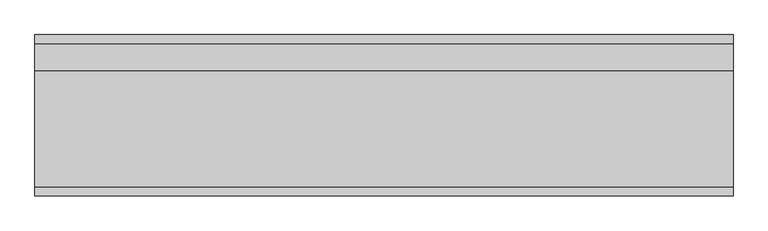
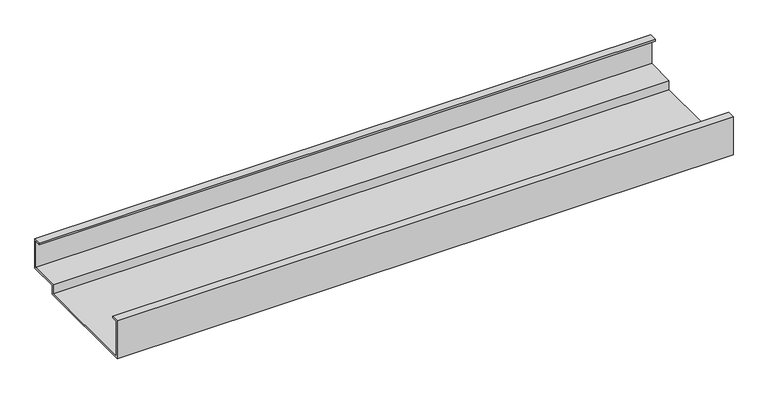
"""IFC4 building model written with IfcOpenShell, lengths in millimetres: proxy geometry, Generic Models 7:Generic Models 1:337419:Generic Models 1:337419 : Generic Models 7:Generic Models 1:337419:13 : Generic Models 7:Generic Models 1:337419:Generic Models 1:337419 : Generic Models 7:Generic Models 1:337419:301336."""

from ifc_helpers import new_model, si_unit, frame, origin, place, context, project, spatial, polyline, outline, extrude, source, transform, mapped, element, save


def generic_models_601f3d41(model_context):
    return source(origin(), model_context, "Body", "SweptSolid", [
        extrude(outline(polyline([(-536557.2913358, 2489.2), (-536557.2913358, 2438.4), (-536606.5038358, 2438.4), (-536606.5038358, 2422.525), (-536792.2413358, 2422.525), (-536792.2413358, 2489.2), (-536779.5413358, 2489.2), (-536779.5413358, 2486.421875), (-536789.4632108, 2486.421875), (-536789.4632108, 2425.303125), (-536609.2819608, 2425.303125), (-536609.2819608, 2441.178125), (-536560.0694608, 2441.178125), (-536560.0694608, 2486.421875), (-536569.9913358, 2486.421875), (-536569.9913358, 2489.2), (-536557.2913358, 2489.2)])), frame((592715.7367242, 0.0, 0.0), z_axis=(1.0, 0.0, 0.0), x_axis=(0.0, 1.0, 0.0)), (0.0, 0.0, 1.0), 1016.0),
    ])


if __name__ == "__main__":
    model = new_model("IFC4")
    model_context = context("Model", 3, world=origin())
    ifc_project = project(units=[si_unit("LENGTHUNIT", "METRE", prefix="MILLI")], contexts=[model_context])
    site = spatial("IfcSite", under=ifc_project)
    building = spatial("IfcBuilding", under=site)
    placement = place(None, origin())
    generic_models_shape = generic_models_601f3d41(model_context)
    element("IfcBuildingElementProxy", 1, Name="Generic Models 7:Generic Models 1:337419:Generic Models 1:337419 : Generic Models 7:Generic Models 1:337419:13 : Generic Models 7:Generic Models 1:337419:Generic Models 1:337419 : Generic Models 7:Generic Models 1:337419:301336", ObjectType="Generic Models 7:Generic Models 1:337419:Generic Models 1:337419 : Generic Models 7:Generic Models 1:337419:13 : Generic Models 7:Generic Models 1:337419:Generic Models 1:337419 : Generic Models 7:Generic Models 1:337419:301336", at=placement, inside=building, context=model_context, shape_type="MappedRepresentation", body=[
        mapped(generic_models_shape, transform((0.0, 0.0, 0.0), x_axis=(1.0, 0.0, 0.0), y_axis=(0.0, 1.0, 0.0), z_axis=(0.0, 0.0, 1.0))),
    ])
    save(model, "model.ifc")

# Revit data of these elements
# Type "Generic Models 7:Generic Models 1:337419:Generic Models 1:337419 : Generic Models 7:Generic Models 1:337419:13 : Generic Models 7:Generic Models 1:337419:Generic Models 1:337419 : Generic Models 7:Generic Models 1:337419:301336"
#   NameOverride = "Generic Models 7:Generic Models 1:337419:Generic Models 1:337419 : Generic Models 7:Generic Models 1:337419:301336"
#   ObjectTypeOverride = "Generic Models 1:337419 : Generic Models 7:Generic Models 1:337419"
#   Reference = "Generic Models 1"
#   Tag = "301336"
# Element 1 (IfcBuildingElementProxy, "Generic Models 7:Generic Models 1:337419:Generic Models 1:337419 : Generic Models 7:Generic Models 1:337419:13 : Generic Models 7:Generic Models 1:337419:Generic Models 1:337419 : Generic Models 7:Generic Models 1:337419:301336")
#   Materials on its faces: "HOLLOW METAL DOOR - SEE DOOR SCHEDULE"
# Materials
#   "HOLLOW METAL DOOR - SEE DOOR SCHEDULE": class "Unassigned", colour RGB 210 209 208, transparency 0, Keynote = "M05121300.02", Cost = 0
